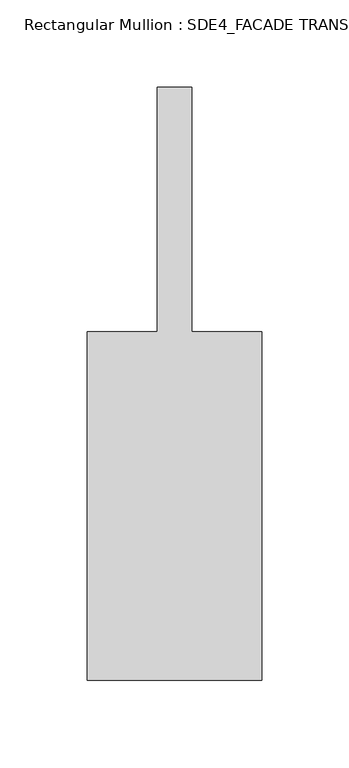
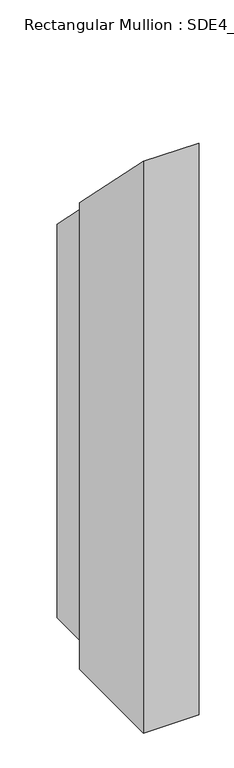
"""IFC4 building model written with IfcOpenShell, lengths in millimetres: member geometry, Rectangular Mullion : SDE4_FACADE TRANSOM TYPE 1."""

from ifc_helpers import new_model, si_unit, origin, place, context, project, spatial, faceted_brep, source, transform, mapped, element, save


def rectangular_mullion_sde4_facade_transom_type_1_5f56726f(model_context):
    return source(origin(), model_context, "Body", "Brep", [
        faceted_brep([(50.0, -132.5, -957.5000001), (-50.0, -132.5, -957.5000001), (-50.0, 67.5, -957.5000001), (-10.0, 67.5, -957.5000001), (-10.0, 207.5, -957.5000001), (10.0, 207.5, -957.5000001), (10.0, 67.5, -957.5000001), (50.0, 67.5, -957.5000001), (50.0, 67.5, -67.5), (50.0, -132.5, 132.5), (10.0, 67.5, -67.5), (10.0, 207.5, -207.5), (-10.0, 207.5, -207.5), (-10.0, 67.5, -67.5), (-50.0, 67.5, -67.5), (-50.0, -132.5, 132.5)], [[[0, 1, 2, 3, 4, 5, 6, 7]], [[8, 9, 0, 7]], [[10, 8, 7, 6]], [[11, 10, 6, 5]], [[12, 11, 5, 4]], [[13, 12, 4, 3]], [[14, 13, 3, 2]], [[15, 14, 2, 1]], [[9, 15, 1, 0]], [[9, 8, 10, 11, 12, 13, 14, 15]]]),
    ])


if __name__ == "__main__":
    model = new_model("IFC4")
    model_context = context("Model", 3, world=origin())
    ifc_project = project(units=[si_unit("LENGTHUNIT", "METRE", prefix="MILLI")], contexts=[model_context])
    site = spatial("IfcSite", under=ifc_project)
    building = spatial("IfcBuilding", under=site)
    placement = place(None, origin())
    rectangular_mullion_sde4_facade_transom_type_1_shape = rectangular_mullion_sde4_facade_transom_type_1_5f56726f(model_context)
    element("IfcMember", 1, ObjectType="Rectangular Mullion : SDE4_FACADE TRANSOM TYPE 1", at=placement, inside=building, context=model_context, shape_type="MappedRepresentation", body=[
        mapped(rectangular_mullion_sde4_facade_transom_type_1_shape, transform((0.0, 0.0, 0.0), x_axis=(1.0, 0.0, 0.0), y_axis=(0.0, 1.0, 0.0), z_axis=(0.0, 0.0, 1.0))),
    ])
    save(model, "model.ifc")

# Revit data of these elements
# Type "Rectangular Mullion : SDE4_FACADE TRANSOM TYPE 1"
#   built-in parameter 1007322 = 1.11549 (stored number, unit not read)
#   built-in parameter 1007321 = 0.164042 (stored number, unit not read)
#   built-in parameter 1007320 = 0.164042 (stored number, unit not read)
